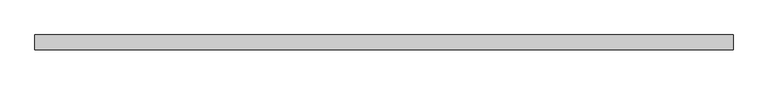
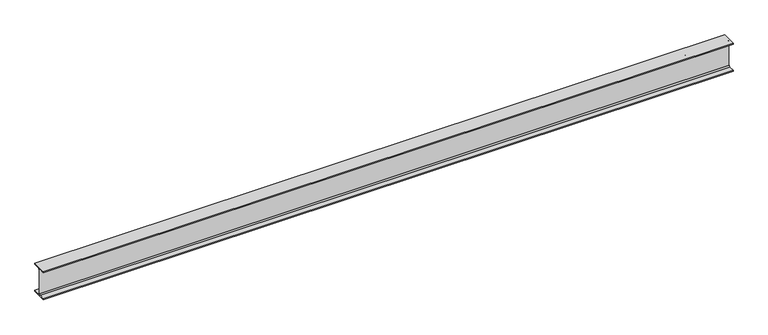
"""IFC4 building model written with IfcOpenShell, lengths in millimetres: beam geometry, 0912_Steel Framing_H-KSD3502 : H_SB_ASB_H-350x175x7x11."""

from ifc_helpers import new_model, si_unit, point, frame, frame_2d, origin, place, context, project, spatial, polyline, circle_curve, trimmed, segment, composite_curve, outline, extrude, source, transform, mapped, element, save


def beam_11403a9d(model_context):
    return source(origin(), model_context, "Body", "SweptSolid", [
        extrude(outline(composite_curve([segment(polyline([(87.5, -164.0), (87.5, -175.0), (-87.5, -175.0), (-87.5, -164.0), (-17.5, -164.0)]), True, "CONTINUOUS"), segment(trimmed(circle_curve(frame_2d((-17.5, -150.0)), 14.0), [point((-17.5, -164.0))], [point((-3.5, -150.0))], True, "CARTESIAN"), True, "CONTINUOUS"), segment(polyline([(-3.5, -150.0), (-3.5, 150.0)]), True, "CONTINUOUS"), segment(trimmed(circle_curve(frame_2d((-17.5, 150.0)), 14.0), [point((-3.5, 150.0))], [point((-17.5, 164.0))], True, "CARTESIAN"), True, "CONTINUOUS"), segment(polyline([(-17.5, 164.0), (-87.5, 164.0), (-87.5, 175.0), (87.5, 175.0), (87.5, 164.0), (17.5, 164.0)]), True, "CONTINUOUS"), segment(trimmed(circle_curve(frame_2d((17.5, 150.0)), 14.0), [point((17.5, 164.0))], [point((3.5, 150.0))], True, "CARTESIAN"), True, "CONTINUOUS"), segment(polyline([(3.5, 150.0), (3.5, -150.0)]), True, "CONTINUOUS"), segment(trimmed(circle_curve(frame_2d((17.5, -150.0)), 14.0), [point((3.5, -150.0))], [point((17.5, -164.0))], True, "CARTESIAN"), True, "CONTINUOUS"), segment(polyline([(17.5, -164.0), (87.5, -164.0)]), True, "CONTINUOUS")], self_intersect=False)), frame((-4087.3, 0.0, 0.0), z_axis=(1.0, 0.0, 0.0), x_axis=(0.0, 1.0, 0.0)), (0.0, 0.0, 1.0), 8174.6),
    ])


if __name__ == "__main__":
    model = new_model("IFC4")
    model_context = context("Model", 3, world=origin())
    ifc_project = project(units=[si_unit("LENGTHUNIT", "METRE", prefix="MILLI")], contexts=[model_context])
    site = spatial("IfcSite", under=ifc_project)
    building = spatial("IfcBuilding", under=site)
    placement = place(None, origin())
    beam_shape = beam_11403a9d(model_context)
    element("IfcBeam", 1, ObjectType="0912_Steel Framing_H-KSD3502 : H_SB_ASB_H-350x175x7x11", at=placement, inside=building, context=model_context, shape_type="MappedRepresentation", body=[
        mapped(beam_shape, transform((0.0, 0.0, 0.0), x_axis=(1.0, 0.0, 0.0), y_axis=(0.0, 1.0, 0.0), z_axis=(0.0, 0.0, 1.0))),
    ])
    save(model, "model.ifc")

# Revit data of these elements
# Type "0912_Steel Framing_H-KSD3502 : H_SB_ASB_H-350x175x7x11"
#   H_WM Code_1 = "S01AA002-00001 | Main Steel Structure Fabrication Work | Shelter/Building | Medium Steel - Standard (90KG/M>Weight≥30KG/M) | Material: (   )"
#   H_WM Code_2 = "S03AA028-00001 | Main Steel Structure Erection Work | Shelter/Building | Medium Steel (90KG/M>Weight≥30KG/M) | Material: (   )"
#   H_WM Code_3 = "S01AA010-00001 | Main Steel Structure Fabrication Work | Shelter/Building | Steel Painting/Coating | for Non-Fireproofed Steel Surface, Surface Preparation, Primer, Second & Final Coat | Material: (   )"
#   H_Q'ty Cal Type Tag = "SB-Q2"
#   Width = 17.5 cm
#   Web Thickness = 0.7 cm
#   Web Fillet = 1.4 cm
#   Warping Constant = 282000.0 cm⁶
#   W = 0
#   Torsional Moment of Inertia = 19.4042 cm⁴
#   Section Area = 63.14 cm²
#   Plastic Modulus weak axis = 174.0 cm³
#   Plastic Modulus strong axis = 868.0 cm³
#   Perimeter = 1.36 m²/m
#   Nominal Weight = 49.60 kgf/m
#   Moment of Inertia weak axis = 984.00 cm⁴
#   Moment of Inertia strong axis = 13600.00 cm⁴
#   Height = 35.0 cm
#   Flange Thickness = 1.1 cm
#   Elastic Modulus weak axis = 112.0 cm³
#   Elastic Modulus strong axis = 775.0 cm³
#   Centroid Vertical = 17.5 cm
#   Centroid Horizontal = 8.75 cm
#   Ix = 136000000
#   Length [instance default] = 1.5240 m
#   Zx = 868000
#   b = 0.1750 m
#   h = 0.3500 m
#   r = 0.0140 m
#   s = 0.0070 m
#   t = 0.0110 m
#   A = 0.006314 m²
#   Structural Material [instance default] = Steel, 45-345
#   Assembly Code = ""
# Element 1 (IfcBeam, "0912_Steel Framing_H-KSD3502 : H_SB_ASB_H-350x175x7x11")
#   Structural Material = none
# Materials
#   "Steel, 45-345": class "Metal", colour RGB 189 187 185, transparency 0, Description = "Steel 345 MPa", Cost = 0
